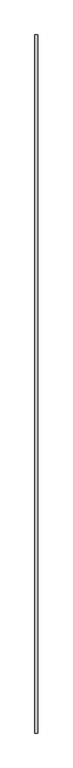
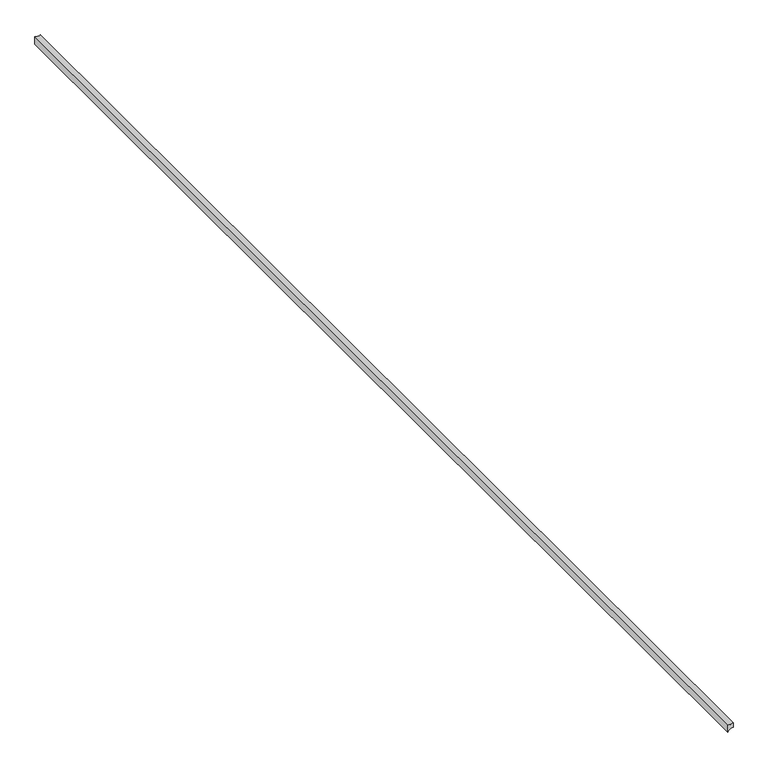
"""IFC4 building model written with IfcOpenShell, lengths in millimetres: proxy geometry, Joint049 8561 : Joint049 8561."""

from ifc_helpers import new_model, si_unit, point, frame, frame_2d, origin, place, context, project, spatial, polyline, circle_curve, trimmed, segment, composite_curve, outline, extrude, source, transform, mapped, element, save


def generic_models_85d0b552(model_context):
    return source(origin(), model_context, "Body", "SweptSolid", [
        extrude(outline(composite_curve([segment(trimmed(circle_curve(frame_2d((39551.0784677, -1997.9402793)), 9.1818164), [point((39554.9304637, -2006.2750185))], [point((39560.2460083, -1997.4284668))], True, "CARTESIAN"), True, "CONTINUOUS"), segment(polyline([(39560.2460083, -1997.4284668), (39568.2455813, -1997.4284668)]), True, "CONTINUOUS"), segment(trimmed(circle_curve(frame_2d((39574.1386556, -2001.8517427)), 7.3684255), [point((39568.2455813, -1997.4284668))], [point((39568.2455813, -2006.2750185))], True, "CARTESIAN"), True, "CONTINUOUS"), segment(polyline([(39568.2455813, -2006.2750185), (39554.9304637, -2006.2750185)]), True, "CONTINUOUS")], self_intersect=False)), frame((0.0, 998.1570038, 0.0), z_axis=(0.0, 1.0, 0.0), x_axis=(0.0, 0.0, 1.0)), (0.0, 0.0, 1.0), 2000.0),
    ])


if __name__ == "__main__":
    model = new_model("IFC4")
    model_context = context("Model", 3, world=origin())
    ifc_project = project(units=[si_unit("LENGTHUNIT", "METRE", prefix="MILLI")], contexts=[model_context])
    site = spatial("IfcSite", under=ifc_project)
    building = spatial("IfcBuilding", under=site)
    placement = place(None, origin())
    generic_models_shape = generic_models_85d0b552(model_context)
    element("IfcBuildingElementProxy", 1, Name="Joint049 8561 : Joint049 8561", ObjectType="Joint049 8561 : Joint049 8561", at=placement, inside=building, context=model_context, shape_type="MappedRepresentation", body=[
        mapped(generic_models_shape, transform((0.0, 0.0, 0.0), x_axis=(1.0, 0.0, 0.0), y_axis=(0.0, 1.0, 0.0), z_axis=(0.0, 0.0, 1.0))),
    ])
    save(model, "model.ifc")

# Revit data of these elements
# Type "Joint049 8561 : Joint049 8561"
#   NameOverride = "Joint049"
# Element 1 (IfcBuildingElementProxy, "Joint049 8561 : Joint049 8561")
#   Materials on its faces: "SEALANT"
# Materials
#   "SEALANT": class "Unassigned", colour RGB 142 225 148, transparency 0
